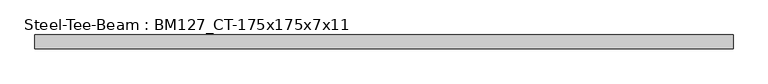
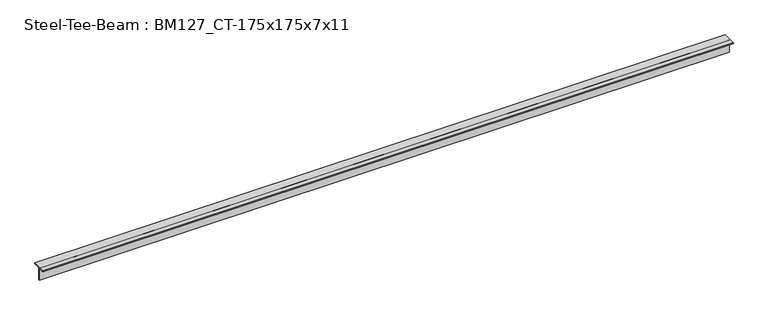
"""IFC4 building model written with IfcOpenShell, lengths in millimetres: beam geometry, Steel-Tee-Beam : BM127_CT-175x175x7x11."""

import ifcopenshell
import ifcopenshell.guid

model = None  # the IFC model being written
_history = None  # IfcOwnerHistory: only IFC2X3 demands one
_inside = {}  # id of a spatial element -> (the spatial element, [elements in it])
_under = {}  # id of a project, library or spatial element -> (it, [spatial elements below it])
_declared = {}  # id of a project -> (the project, [libraries it declares])
_typed = {}  # id of a type object -> (the type object, [elements of that type])
_made_of = {}  # id of a material, layer set ... -> (it, [elements and type objects made of it])


def new_model(schema):
    """Start an empty IFC model of exactly this schema.

    Asked for "IFC4X3", IfcOpenShell would pick the latest addendum, in which some entities
    have other attributes; the version numbers below select the first issue.
    IFC2X3 requires an IfcOwnerHistory on every rooted entity: one is made here for all.
    """
    global model, _history
    if schema == "IFC4X3":
        model = ifcopenshell.file(schema_version=(4, 3, 0, 0))
    else:
        model = ifcopenshell.file(schema=schema)
    _inside.clear()
    _under.clear()
    _declared.clear()
    _typed.clear()
    _made_of.clear()
    _history = None
    if model.schema == "IFC2X3":
        org = make("IfcOrganization", Name="unknown")
        user = make(
            "IfcPersonAndOrganization",
            ThePerson=make("IfcPerson", FamilyName="unknown"),
            TheOrganization=org,
        )
        app = make(
            "IfcApplication",
            ApplicationDeveloper=org,
            Version="unknown",
            ApplicationFullName="unknown",
            ApplicationIdentifier="unknown",
        )
        _history = make(
            "IfcOwnerHistory",
            OwningUser=user,
            OwningApplication=app,
            ChangeAction="ADDED",
            CreationDate=0,
        )
    return model


def make(cls, **values):
    """One entity of the class cls with the attributes given. An attribute that is None is left unset."""
    return model.create_entity(
        cls, **{name: value for name, value in values.items() if value is not None}
    )


def rooted(cls, **values):
    """An entity with a GlobalId (a new one), such as an element, a storey or a relation."""
    return make(cls, GlobalId=ifcopenshell.guid.new(), OwnerHistory=_history, **values)


def si_unit(unit_type, name, prefix=None):
    """IfcSIUnit, for example si_unit("LENGTHUNIT", "METRE", prefix="MILLI")."""
    return make("IfcSIUnit", UnitType=unit_type, Prefix=prefix, Name=name)


def assignment(units):
    """IfcUnitAssignment: the units of a project."""
    return None if units is None else make("IfcUnitAssignment", Units=units)


def point(xyz):
    """IfcCartesianPoint."""
    return None if xyz is None else make("IfcCartesianPoint", Coordinates=xyz)


def direction(xyz):
    """IfcDirection."""
    return None if xyz is None else make("IfcDirection", DirectionRatios=xyz)


def frame(location, z_axis=None, x_axis=None):
    """IfcAxis2Placement3D, a coordinate frame: its origin and axes. An axis left out is left unset."""
    return make(
        "IfcAxis2Placement3D",
        Location=point(location),
        Axis=direction(z_axis),
        RefDirection=direction(x_axis),
    )


def frame_2d(location, x_axis=None):
    """IfcAxis2Placement2D, a coordinate frame in the plane: its origin and x axis."""
    return make(
        "IfcAxis2Placement2D", Location=point(location), RefDirection=direction(x_axis)
    )


def origin():
    """The frame at (0, 0, 0) with its axes left unset."""
    return frame((0.0, 0.0, 0.0))


def place(relative_to, where):
    """IfcLocalPlacement: puts the frame where relative to a parent placement (None: the world)."""
    return make(
        "IfcLocalPlacement", PlacementRelTo=relative_to, RelativePlacement=where
    )


def context(
    kind, dimensions, precision=None, world=None, true_north=None, identifier=None
):
    """IfcGeometricRepresentationContext, for example the 3D "Model" context."""
    return make(
        "IfcGeometricRepresentationContext",
        ContextIdentifier=identifier,
        ContextType=kind,
        CoordinateSpaceDimension=dimensions,
        Precision=precision,
        WorldCoordinateSystem=world,
        TrueNorth=true_north,
    )


def project(units=None, contexts=None):
    """IfcProject with its units and contexts."""
    return rooted(
        "IfcProject",
        Name="project",
        RepresentationContexts=contexts,
        UnitsInContext=assignment(units),
    )


def spatial(cls, under=None, at=None, **own):
    """A site, building, storey or space (cls), placed at a placement, below another one or the project."""
    s = rooted(cls, ObjectPlacement=at, **own)
    if under is not None:
        _under.setdefault(under.id(), (under, []))[1].append(s)
    return s


def polyline(points):
    """IfcPolyline through the points."""
    return make("IfcPolyline", Points=[point(p) for p in points])


def circle_curve(where, radius):
    """IfcCircle in the frame where."""
    return make("IfcCircle", Position=where, Radius=radius)


def trimmed(basis, trim1, trim2, sense, master):
    """IfcTrimmedCurve: the piece of a basis curve between two trims."""
    return make(
        "IfcTrimmedCurve",
        BasisCurve=basis,
        Trim1=trim1,
        Trim2=trim2,
        SenseAgreement=sense,
        MasterRepresentation=master,
    )


def segment(curve, same_sense, transition):
    """IfcCompositeCurveSegment."""
    return make(
        "IfcCompositeCurveSegment",
        Transition=transition,
        SameSense=same_sense,
        ParentCurve=curve,
    )


def composite_curve(segments, self_intersect=None):
    """IfcCompositeCurve: segments joined end to end."""
    return make("IfcCompositeCurve", Segments=segments, SelfIntersect=self_intersect)


def outline(outer, holes=None, kind="AREA"):
    """IfcArbitraryClosedProfileDef: a profile drawn as a closed curve; with holes, ...WithVoids."""
    if holes is None:
        return make("IfcArbitraryClosedProfileDef", ProfileType=kind, OuterCurve=outer)
    return make(
        "IfcArbitraryProfileDefWithVoids",
        ProfileType=kind,
        OuterCurve=outer,
        InnerCurves=holes,
    )


def extrude(swept, where, along, depth):
    """IfcExtrudedAreaSolid: the profile swept, set in the frame where, extruded along a direction by depth."""
    return make(
        "IfcExtrudedAreaSolid",
        SweptArea=swept,
        Position=where,
        ExtrudedDirection=direction(along),
        Depth=depth,
    )


def shape(context_of_items, identifier, shape_type, items):
    """IfcShapeRepresentation: the items that make up one representation, for example the "Body"."""
    return make(
        "IfcShapeRepresentation",
        ContextOfItems=context_of_items,
        RepresentationIdentifier=identifier,
        RepresentationType=shape_type,
        Items=items,
    )


def source(mapping_origin, context_of_items, identifier, shape_type, items):
    """IfcRepresentationMap: a shape defined once, which mapped items show again and again."""
    return make(
        "IfcRepresentationMap",
        MappingOrigin=mapping_origin,
        MappedRepresentation=shape(context_of_items, identifier, shape_type, items),
    )


def transform(
    local_origin,
    x_axis=None,
    y_axis=None,
    z_axis=None,
    scale=None,
    scale2=None,
    scale3=None,
    uniform=True,
):
    """IfcCartesianTransformationOperator3D, or its non-uniform kind. x_axis, y_axis, z_axis: its Axis1, 2, 3."""
    if uniform:
        return make(
            "IfcCartesianTransformationOperator3D",
            Axis1=direction(x_axis),
            Axis2=direction(y_axis),
            LocalOrigin=point(local_origin),
            Scale=scale,
            Axis3=direction(z_axis),
        )
    return make(
        "IfcCartesianTransformationOperator3DnonUniform",
        Axis1=direction(x_axis),
        Axis2=direction(y_axis),
        LocalOrigin=point(local_origin),
        Scale=scale,
        Axis3=direction(z_axis),
        Scale2=scale2,
        Scale3=scale3,
    )


def mapped(mapping_source, mapping_target):
    """IfcMappedItem: shows the shape of a source again, moved by a transform."""
    return make(
        "IfcMappedItem", MappingSource=mapping_source, MappingTarget=mapping_target
    )


def made_of(thing, what):
    """Note that an element or type object is made of a material, layer set ...; save() writes the relation."""
    if what is not None:
        _made_of.setdefault(what.id(), (what, []))[1].append(thing)
    return thing


def element(
    cls,
    number,
    at=None,
    inside=None,
    cuts=None,
    type_object=None,
    material=None,
    context=None,
    identifier="Body",
    shape_type=None,
    held_by="IfcProductDefinitionShape",
    body=None,
    shapes=None,
    **own,
):
    """One element of the class cls, such as IfcWall. Its Tag is "e" and its number.

    at: its placement. inside: the storey or other place that contains it. cuts: it is an
    opening in that element (IfcRelVoidsElement). A single representation is given by context,
    identifier, shape_type and body (its items); several are given by shapes. held_by: the class
    of the entity that holds the representations. save() writes the other relations.
    """
    e = rooted(cls, Tag="e%d" % number, ObjectPlacement=at, **own)
    if body is not None:
        shapes = [shape(context, identifier, shape_type, body)]
    if shapes is not None:
        e.Representation = make(held_by, Representations=shapes)
    if inside is not None:
        _inside.setdefault(inside.id(), (inside, []))[1].append(e)
    if cuts is not None:
        rooted(
            "IfcRelVoidsElement", RelatingBuildingElement=cuts, RelatedOpeningElement=e
        )
    if type_object is not None:
        _typed.setdefault(type_object.id(), (type_object, []))[1].append(e)
    return made_of(e, material)


def aggregate(whole, parts):
    """IfcRelAggregates: a whole, such as a stair, and the parts it consists of."""
    return rooted("IfcRelAggregates", RelatingObject=whole, RelatedObjects=parts)


def save(model, path):
    """Write the relations noted so far, then the file.

    IfcRelAggregates (storeys below a building ...), IfcRelContainedInSpatialStructure (elements
    in a storey), IfcRelDefinesByType, IfcRelAssociatesMaterial and IfcRelDeclares: one each for
    every whole, place, type object, material and project.
    """
    for whole, parts in _under.values():
        aggregate(whole, parts)
    for where, things in _inside.values():
        rooted(
            "IfcRelContainedInSpatialStructure",
            RelatedElements=things,
            RelatingStructure=where,
        )
    for kind, things in _typed.values():
        rooted("IfcRelDefinesByType", RelatedObjects=things, RelatingType=kind)
    for what, things in _made_of.values():
        rooted("IfcRelAssociatesMaterial", RelatedObjects=things, RelatingMaterial=what)
    for by, libraries in _declared.values():
        rooted("IfcRelDeclares", RelatingContext=by, RelatedDefinitions=libraries)
    model.write(path)


def steel_tee_beam_bm127_ct_175x175x7x11_7511bb12(model_context):
    return source(origin(), model_context, "Body", "SweptSolid", [
        extrude(outline(composite_curve([segment(polyline([(87.5, 87.5), (87.5, 76.5), (17.5, 76.5)]), True, "CONTINUOUS"), segment(trimmed(circle_curve(frame_2d((17.5, 62.5)), 14.0), [point((17.5, 76.5))], [point((3.5, 62.5))], True, "CARTESIAN"), True, "CONTINUOUS"), segment(polyline([(3.5, 62.5), (3.5, -87.5), (-3.5, -87.5), (-3.5, 62.5)]), True, "CONTINUOUS"), segment(trimmed(circle_curve(frame_2d((-17.5, 62.5)), 14.0), [point((-3.5, 62.5))], [point((-17.5, 76.5))], True, "CARTESIAN"), True, "CONTINUOUS"), segment(polyline([(-17.5, 76.5), (-87.5, 76.5), (-87.5, 87.5), (87.5, 87.5)]), True, "CONTINUOUS")], self_intersect=False)), frame((-4427.0238227, 0.0, 0.0), z_axis=(1.0, 0.0, 0.0), x_axis=(0.0, 1.0, 0.0)), (0.0, 0.0, 1.0), 8723.5825238),
    ])


if __name__ == "__main__":
    model = new_model("IFC4")
    model_context = context("Model", 3, world=origin())
    ifc_project = project(units=[si_unit("LENGTHUNIT", "METRE", prefix="MILLI")], contexts=[model_context])
    site = spatial("IfcSite", under=ifc_project)
    building = spatial("IfcBuilding", under=site)
    placement = place(None, origin())
    steel_tee_beam_bm127_ct_175x175x7x11_shape = steel_tee_beam_bm127_ct_175x175x7x11_7511bb12(model_context)
    element("IfcBeam", 1, ObjectType="Steel-Tee-Beam : BM127_CT-175x175x7x11", at=placement, inside=building, context=model_context, shape_type="MappedRepresentation", body=[
        mapped(steel_tee_beam_bm127_ct_175x175x7x11_shape, transform((0.0, 0.0, 0.0), x_axis=(1.0, 0.0, 0.0), y_axis=(0.0, 1.0, 0.0), z_axis=(0.0, 0.0, 1.0))),
    ])
    save(model, "model.ifc")

# Revit data of these elements
# Type "Steel-Tee-Beam : BM127_CT-175x175x7x11"
#   Surface Area = 0.687982 m²/m
#   Section Area = 31.5712 cm²
#   Mass per Unit Length = 24.7834 kg/m
#   Length [instance default] = 1524 mm
#   bf = 175 mm
#   d = 175 mm
#   k = 25 mm
#   r = 14 mm
#   tf = 11 mm
#   tw = 7 mm
#   hec_material4 [instance default] = none
#   hec_material3 [instance default] = none
#   hec_material2 [instance default] = none
#   hec_material1 [instance default] = none
#   Structural Material [instance default] = Steel, 45-345
#   Assembly Code = ""
# Element 1 (IfcBeam, "Steel-Tee-Beam : BM127_CT-175x175x7x11")
#   hec_material3 = F01AC000-00002_Building/Shelter Fire Proofing Work_Intumescent Coating Type_1 hr. rating (UL 1709))
#   hec_material2 = S01AA010-00002_Main Steel Structure Fabrication Work_Shelter/Building_Steel Painting/Coating_for Fireproofed Steel Surface, Surface Preparation & Primer Coat
#   hec_material1 = S03AA029-00001_Main Steel Structure Erection Work_Shelter/Building_Light Steel
#   Structural Material = S01AA003-00001_Main Steel Structure Fabrication Work_Shelter/Building_Light Steel - Standard
#   Materials on its faces: "S01AA003-00001_Main Steel Structure Fabrication Work_Shelter/Building_Light Steel - Standard"
# Materials
#   "Steel, 45-345": class "Metal", colour RGB 189 187 185, transparency 0, Description = "Steel 345 MPa", Cost = 0
#   "S01AA003-00001_Main Steel Structure Fabrication Work_Shelter/Building_Light Steel - Standard": class "Metal", colour RGB 120 120 120, transparency 0, Comments = "(30KG/M>Weight)", Description = "Structural steel 50ksi", W00) Work Master Code = "S01AA003-00001", W01) Work Master_Lv1 = "Main Steel Structure Fabrication Work", W02) Work Master_Lv2 = "Shelter/Building", W03) Work Master_Spec.1 = "Light Steel - Standard (30KG/M>Weight)", Cost = 0
#   "F01AC000-00002_Building/Shelter Fire Proofing Work_Intumescent Coating Type_1 hr. rating (UL 1709))": class "Metal", colour RGB 255 128 128, transparency 0, Description = "Paint finished steel", W00) Work Master Code = "F01AC000-00002", W01) Work Master_Lv1 = "Building/Shelter Fire Proofing Work", W02) Work Master_Lv2 = "Intumescent Coating Type", W03) Work Master_Spec.1 = "1 hr. rating (UL 1709)", Cost = 0
#   "S01AA010-00002_Main Steel Structure Fabrication Work_Shelter/Building_Steel Painting/Coating_for Fireproofed Steel Surface, Surface Preparation & Primer Coat": class "Metal", colour RGB 120 120 120, transparency 0, Description = "Paint finished steel", W00) Work Master Code = "SS01AA010-00002", W01) Work Master_Lv1 = "Main Steel Structure Fabrication Work", W02) Work Master_Lv2 = "Shelter/Building", W03) Work Master_Spec.1 = "Steel Painting/Coating", W04) Work Master_Spec.2 = "for Fireproofed Steel Surface, Surface Preparation & Primer Coat", Cost = 0
#   "S03AA029-00001_Main Steel Structure Erection Work_Shelter/Building_Light Steel": class "Metal", colour RGB 120 120 120, transparency 0, Comments = "(30KG/M>Weight)", Description = "Structural steel 50ksi", W00) Work Master Code = "S03AA029-00001", W01) Work Master_Lv1 = "Main Steel Structure Erection Work", W02) Work Master_Lv2 = "Shelter/Building", W03) Work Master_Spec.1 = "Light Steel (30KG/M>Weight)", Cost = 0
